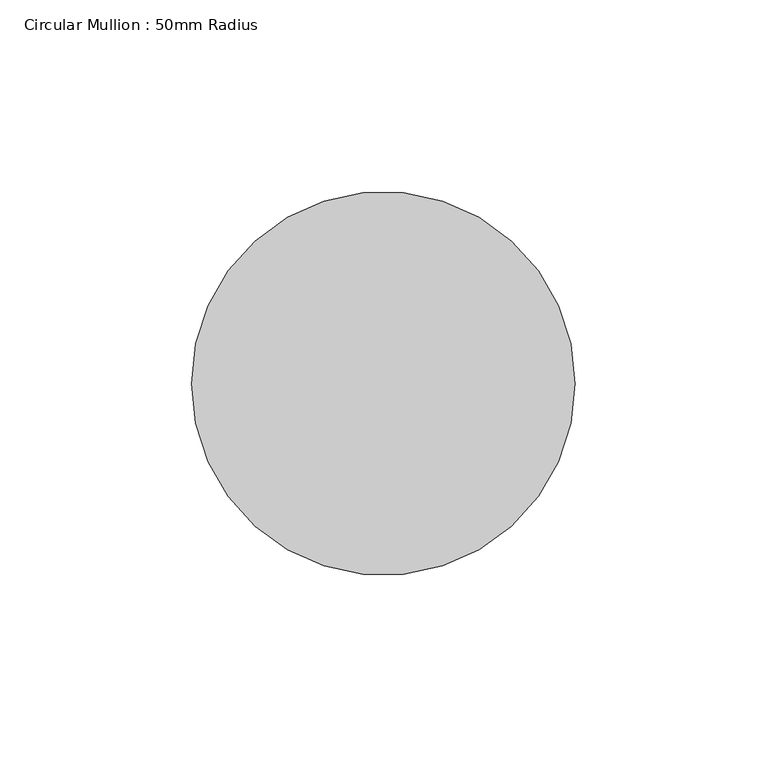
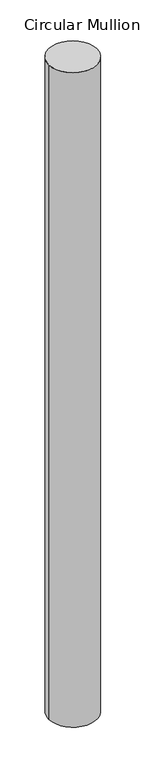
"""IFC4 building model written with IfcOpenShell, lengths in millimetres: member geometry, Circular Mullion : 50mm Radius."""

from ifc_helpers import new_model, si_unit, point, frame, origin, origin_2d, place, context, project, spatial, circle_curve, trimmed, segment, composite_curve, outline, extrude, source, transform, mapped, element, save


def circular_mullion_50mm_radius_01a66951(model_context):
    return source(origin(), model_context, "Body", "SweptSolid", [
        extrude(outline(composite_curve([segment(trimmed(circle_curve(origin_2d(), 50.0), [point((50.0, 0.0))], [point((-50.0, 0.0))], False, "CARTESIAN"), True, "CONTINUOUS"), segment(trimmed(circle_curve(origin_2d(), 50.0), [point((-50.0, 0.0))], [point((50.0, 0.0))], False, "CARTESIAN"), True, "CONTINUOUS")], self_intersect=False)), frame((0.0, 0.0, -1430.1071754), z_axis=(0.0, 0.0, 1.0), x_axis=(1.0, 0.0, 0.0)), (0.0, 0.0, 1.0), 1430.1071754),
    ])


if __name__ == "__main__":
    model = new_model("IFC4")
    model_context = context("Model", 3, world=origin())
    ifc_project = project(units=[si_unit("LENGTHUNIT", "METRE", prefix="MILLI")], contexts=[model_context])
    site = spatial("IfcSite", under=ifc_project)
    building = spatial("IfcBuilding", under=site)
    placement = place(None, origin())
    circular_mullion_50mm_radius_shape = circular_mullion_50mm_radius_01a66951(model_context)
    element("IfcMember", 1, ObjectType="Circular Mullion : 50mm Radius", at=placement, inside=building, context=model_context, shape_type="MappedRepresentation", body=[
        mapped(circular_mullion_50mm_radius_shape, transform((0.0, 0.0, 0.0), x_axis=(1.0, 0.0, 0.0), y_axis=(0.0, 1.0, 0.0), z_axis=(0.0, 0.0, 1.0))),
    ])
    save(model, "model.ifc")

# Revit data of these elements
# Type "Circular Mullion : 50mm Radius"
#   built-in parameter 1007350 = 0.164042 (stored number, unit not read)
# Element 1 (IfcMember, "Circular Mullion : 50mm Radius")
#   Materials on its faces: "Aluminium"
# Materials
#   "Aluminium": class "Metal", colour RGB 247 247 247, transparency 0, Description = "Aluminium 6061", Cost = 0
